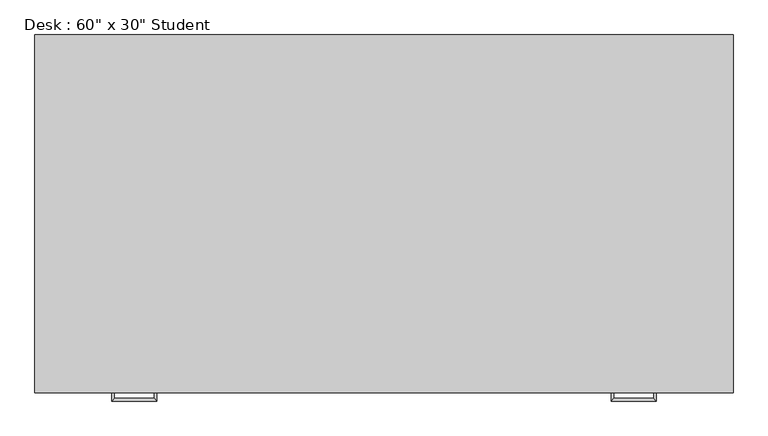
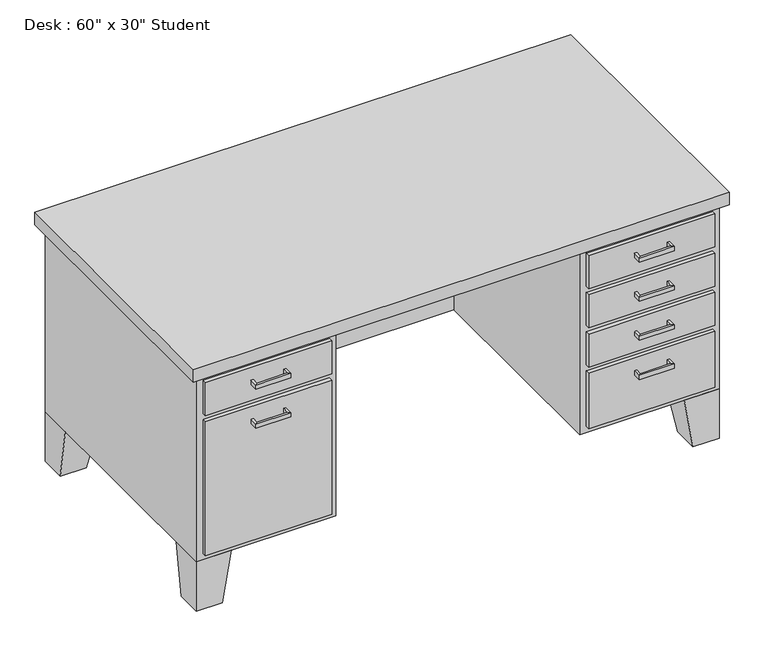
"""IFC4 building model written with IfcOpenShell, lengths in millimetres: furniture geometry."""

from ifc_helpers import new_model, si_unit, frame, origin, place, context, project, spatial, polyline, outline, extrude, faceted_brep, source, transform, mapped, element, save


def furniture_0f337a0f(model_context):
    return source(origin(), model_context, "Body", "SolidModel", [
        extrude(outline(polyline([(1117.6, 0.0), (1117.6, 635.0), (406.4, 635.0), (406.4, 0.0), (0.0, 0.0), (0.0, 762.0), (1524.0, 762.0), (1524.0, 0.0), (1117.6, 0.0)])), frame((0.0, 0.0, 152.4), z_axis=(0.0, 0.0, 1.0), x_axis=(1.0, 0.0, 0.0)), (0.0, 0.0, 1.0), 571.5),
        extrude(outline(polyline([(-19.05, -19.05), (-19.05, 781.05), (1543.05, 781.05), (1543.05, -19.05), (-19.05, -19.05)])), frame((0.0, 0.0, 723.9), z_axis=(0.0, 0.0, 1.0), x_axis=(1.0, 0.0, 0.0)), (0.0, 0.0, 1.0), 38.1),
        faceted_brep([(1422.4, 0.0, 152.4), (1524.0, 0.0, 152.4), (1524.0, 101.6, 152.4), (1422.4, 101.6, 152.4), (1447.8, 0.0, 0.0), (1447.8, 76.2, 0.0), (1524.0, 76.2, 0.0), (1524.0, 0.0, 0.0)], [[[0, 1, 2, 3]], [[4, 5, 6, 7]], [[4, 7, 1, 0]], [[7, 6, 2, 1]], [[6, 5, 3, 2]], [[5, 4, 0, 3]]]),
        faceted_brep([(1422.4, 762.0, 152.4), (1422.4, 660.4, 152.4), (1524.0, 660.4, 152.4), (1524.0, 762.0, 152.4), (1447.8, 762.0, 0.0), (1524.0, 762.0, 0.0), (1524.0, 685.8, 0.0), (1447.8, 685.8, 0.0)], [[[0, 1, 2, 3]], [[4, 5, 6, 7]], [[4, 7, 1, 0]], [[7, 6, 2, 1]], [[6, 5, 3, 2]], [[5, 4, 0, 3]]]),
        faceted_brep([(101.6, 762.0, 152.4), (0.0, 762.0, 152.4), (0.0, 660.4, 152.4), (101.6, 660.4, 152.4), (76.2, 762.0, 0.0), (76.2, 685.8, 0.0), (0.0, 685.8, 0.0), (0.0, 762.0, 0.0)], [[[0, 1, 2, 3]], [[4, 5, 6, 7]], [[4, 7, 1, 0]], [[7, 6, 2, 1]], [[6, 5, 3, 2]], [[5, 4, 0, 3]]]),
        faceted_brep([(101.6, 0.0, 152.4), (101.6, 101.6, 152.4), (0.0, 101.6, 152.4), (0.0, 0.0, 152.4), (76.2, 0.0, 0.0), (0.0, 0.0, 0.0), (0.0, 76.2, 0.0), (76.2, 76.2, 0.0)], [[[0, 1, 2, 3]], [[4, 5, 6, 7]], [[4, 7, 1, 0]], [[7, 6, 2, 1]], [[6, 5, 3, 2]], [[5, 4, 0, 3]]]),
        extrude(outline(polyline([(1136.65, 0.0), (1504.95, 0.0), (1504.95, -12.7), (1136.65, -12.7), (1136.65, 0.0)])), frame((0.0, 0.0, 603.25), z_axis=(0.0, 0.0, 1.0), x_axis=(1.0, 0.0, 0.0)), (0.0, 0.0, 1.0), 101.6),
        extrude(outline(polyline([(1136.65, 0.0), (1504.95, 0.0), (1504.95, -12.7), (1136.65, -12.7), (1136.65, 0.0)])), frame((0.0, 0.0, 171.45), z_axis=(0.0, 0.0, 1.0), x_axis=(1.0, 0.0, 0.0)), (0.0, 0.0, 1.0), 171.45),
        extrude(outline(polyline([(1136.65, 0.0), (1504.95, 0.0), (1504.95, -12.7), (1136.65, -12.7), (1136.65, 0.0)])), frame((0.0, 0.0, 482.6), z_axis=(0.0, 0.0, 1.0), x_axis=(1.0, 0.0, 0.0)), (0.0, 0.0, 1.0), 101.6),
        extrude(outline(polyline([(1136.65, 0.0), (1504.95, 0.0), (1504.95, -12.7), (1136.65, -12.7), (1136.65, 0.0)])), frame((0.0, 0.0, 361.95), z_axis=(0.0, 0.0, 1.0), x_axis=(1.0, 0.0, 0.0)), (0.0, 0.0, 1.0), 101.6),
        extrude(outline(polyline([(19.05, 0.0), (387.35, 0.0), (387.35, -12.7), (19.05, -12.7), (19.05, 0.0)])), frame((0.0, 0.0, 603.25), z_axis=(0.0, 0.0, 1.0), x_axis=(1.0, 0.0, 0.0)), (0.0, 0.0, 1.0), 101.6),
        extrude(outline(polyline([(19.05, 0.0), (387.35, 0.0), (387.35, -12.7), (19.05, -12.7), (19.05, 0.0)])), frame((0.0, 0.0, 171.45), z_axis=(0.0, 0.0, 1.0), x_axis=(1.0, 0.0, 0.0)), (0.0, 0.0, 1.0), 412.75),
        faceted_brep([(1365.25, -12.7, 304.8), (1371.6, -12.7, 304.8), (1371.6, -12.7, 292.1), (1365.25, -12.7, 292.1), (1365.25, -31.75, 304.8), (1371.6, -38.1, 304.8), (1371.6, -38.1, 292.1), (1365.25, -31.75, 292.1), (1276.35, -31.75, 304.8), (1270.0, -38.1, 304.8), (1270.0, -38.1, 292.1), (1276.35, -31.75, 292.1), (1276.35, -12.7, 304.8), (1276.35, -12.7, 292.1), (1270.0, -12.7, 292.1), (1270.0, -12.7, 304.8)], [[[0, 1, 2, 3]], [[1, 0, 4, 5]], [[2, 1, 5, 6]], [[3, 2, 6, 7]], [[0, 3, 7, 4]], [[5, 4, 8, 9]], [[6, 5, 9, 10]], [[7, 6, 10, 11]], [[4, 7, 11, 8]], [[12, 13, 14, 15]], [[9, 8, 12, 15]], [[10, 9, 15, 14]], [[11, 10, 14, 13]], [[8, 11, 13, 12]]]),
        faceted_brep([(1365.25, -12.7, 425.45), (1371.6, -12.7, 425.45), (1371.6, -12.7, 412.75), (1365.25, -12.7, 412.75), (1365.25, -31.75, 425.45), (1371.6, -38.1, 425.45), (1371.6, -38.1, 412.75), (1365.25, -31.75, 412.75), (1276.35, -31.75, 425.45), (1270.0, -38.1, 425.45), (1270.0, -38.1, 412.75), (1276.35, -31.75, 412.75), (1276.35, -12.7, 425.45), (1276.35, -12.7, 412.75), (1270.0, -12.7, 412.75), (1270.0, -12.7, 425.45)], [[[0, 1, 2, 3]], [[1, 0, 4, 5]], [[2, 1, 5, 6]], [[3, 2, 6, 7]], [[0, 3, 7, 4]], [[5, 4, 8, 9]], [[6, 5, 9, 10]], [[7, 6, 10, 11]], [[4, 7, 11, 8]], [[12, 13, 14, 15]], [[9, 8, 12, 15]], [[10, 9, 15, 14]], [[11, 10, 14, 13]], [[8, 11, 13, 12]]]),
        faceted_brep([(1365.25, -12.7, 546.1), (1371.6, -12.7, 546.1), (1371.6, -12.7, 533.4), (1365.25, -12.7, 533.4), (1365.25, -31.75, 546.1), (1371.6, -38.1, 546.1), (1371.6, -38.1, 533.4), (1365.25, -31.75, 533.4), (1276.35, -31.75, 546.1), (1270.0, -38.1, 546.1), (1270.0, -38.1, 533.4), (1276.35, -31.75, 533.4), (1276.35, -12.7, 546.1), (1276.35, -12.7, 533.4), (1270.0, -12.7, 533.4), (1270.0, -12.7, 546.1)], [[[0, 1, 2, 3]], [[1, 0, 4, 5]], [[2, 1, 5, 6]], [[3, 2, 6, 7]], [[0, 3, 7, 4]], [[5, 4, 8, 9]], [[6, 5, 9, 10]], [[7, 6, 10, 11]], [[4, 7, 11, 8]], [[12, 13, 14, 15]], [[9, 8, 12, 15]], [[10, 9, 15, 14]], [[11, 10, 14, 13]], [[8, 11, 13, 12]]]),
        faceted_brep([(1365.25, -12.7, 666.75), (1371.6, -12.7, 666.75), (1371.6, -12.7, 654.05), (1365.25, -12.7, 654.05), (1365.25, -31.75, 666.75), (1371.6, -38.1, 666.75), (1371.6, -38.1, 654.05), (1365.25, -31.75, 654.05), (1276.35, -31.75, 666.75), (1270.0, -38.1, 666.75), (1270.0, -38.1, 654.05), (1276.35, -31.75, 654.05), (1276.35, -12.7, 666.75), (1276.35, -12.7, 654.05), (1270.0, -12.7, 654.05), (1270.0, -12.7, 666.75)], [[[0, 1, 2, 3]], [[1, 0, 4, 5]], [[2, 1, 5, 6]], [[3, 2, 6, 7]], [[0, 3, 7, 4]], [[5, 4, 8, 9]], [[6, 5, 9, 10]], [[7, 6, 10, 11]], [[4, 7, 11, 8]], [[12, 13, 14, 15]], [[9, 8, 12, 15]], [[10, 9, 15, 14]], [[11, 10, 14, 13]], [[8, 11, 13, 12]]]),
        faceted_brep([(158.75, -12.7, 546.1), (158.75, -12.7, 533.4), (152.4, -12.7, 533.4), (152.4, -12.7, 546.1), (158.75, -31.75, 546.1), (158.75, -31.75, 533.4), (152.4, -38.1, 533.4), (152.4, -38.1, 546.1), (247.65, -31.75, 546.1), (247.65, -31.75, 533.4), (254.0, -38.1, 533.4), (254.0, -38.1, 546.1), (247.65, -12.7, 546.1), (254.0, -12.7, 546.1), (254.0, -12.7, 533.4), (247.65, -12.7, 533.4)], [[[0, 1, 2, 3]], [[1, 0, 4, 5]], [[2, 1, 5, 6]], [[3, 2, 6, 7]], [[0, 3, 7, 4]], [[5, 4, 8, 9]], [[6, 5, 9, 10]], [[7, 6, 10, 11]], [[4, 7, 11, 8]], [[12, 13, 14, 15]], [[9, 8, 12, 15]], [[10, 9, 15, 14]], [[11, 10, 14, 13]], [[8, 11, 13, 12]]]),
        faceted_brep([(158.75, -12.7, 666.75), (158.75, -12.7, 654.05), (152.4, -12.7, 654.05), (152.4, -12.7, 666.75), (158.75, -31.75, 666.75), (158.75, -31.75, 654.05), (152.4, -38.1, 654.05), (152.4, -38.1, 666.75), (247.65, -31.75, 666.75), (247.65, -31.75, 654.05), (254.0, -38.1, 654.05), (254.0, -38.1, 666.75), (247.65, -12.7, 666.75), (254.0, -12.7, 666.75), (254.0, -12.7, 654.05), (247.65, -12.7, 654.05)], [[[0, 1, 2, 3]], [[1, 0, 4, 5]], [[2, 1, 5, 6]], [[3, 2, 6, 7]], [[0, 3, 7, 4]], [[5, 4, 8, 9]], [[6, 5, 9, 10]], [[7, 6, 10, 11]], [[4, 7, 11, 8]], [[12, 13, 14, 15]], [[9, 8, 12, 15]], [[10, 9, 15, 14]], [[11, 10, 14, 13]], [[8, 11, 13, 12]]]),
    ])


if __name__ == "__main__":
    model = new_model("IFC4")
    model_context = context("Model", 3, world=origin())
    ifc_project = project(units=[si_unit("LENGTHUNIT", "METRE", prefix="MILLI")], contexts=[model_context])
    site = spatial("IfcSite", under=ifc_project)
    building = spatial("IfcBuilding", under=site)
    placement = place(None, origin())
    furniture_shape = furniture_0f337a0f(model_context)
    element("IfcFurniture", 1, ObjectType="Desk : 60\" x 30\" Student", at=placement, inside=building, context=model_context, shape_type="MappedRepresentation", body=[
        mapped(furniture_shape, transform((0.0, 0.0, 0.0), x_axis=(1.0, 0.0, 0.0), y_axis=(0.0, 1.0, 0.0), z_axis=(0.0, 0.0, 1.0))),
    ])
    save(model, "model.ifc")

# Revit data of these elements
# Type "Desk : 60\" x 30\" Student"
#   Assembly Code = "E2020200"
#   Depth = 2' - 6"
#   Height = 2' - 6"
#   Leg Height = 0' - 6"
#   Width = 5' - 0"
#   Body Material = Laminate, Ivory, Matte
#   Handle/Leg Material = Steel, Chrome Plated
#   Top Material = Cherry
#   Default Elevation = 0
# Element 1 (IfcFurniture, "Desk : 60\" x 30\" Student")
#   Materials on its faces: "Steel, Chrome Plated", "Laminate, Ivory, Matte", "Cherry"
# Materials
#   "Laminate, Ivory, Matte": class "Plastic", colour RGB 247 247 239, transparency 0, Description = "Plastic Laminate - Ivory, Matte", Cost = 0
#   "Steel, Chrome Plated": class "Metal", colour RGB 244 244 244, transparency 0, Description = "Chromiuim plated steel", Cost = 0
#   "Cherry": class "Wood", colour RGB 233 182 144, transparency 0, Description = "Prunus Serotina", Cost = 0
